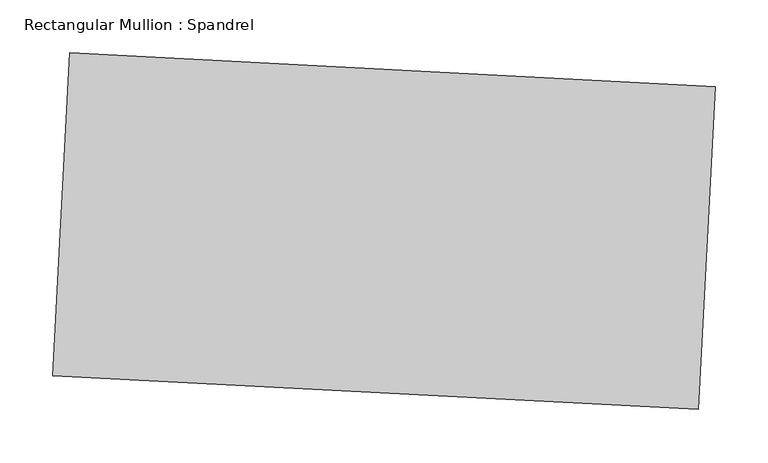
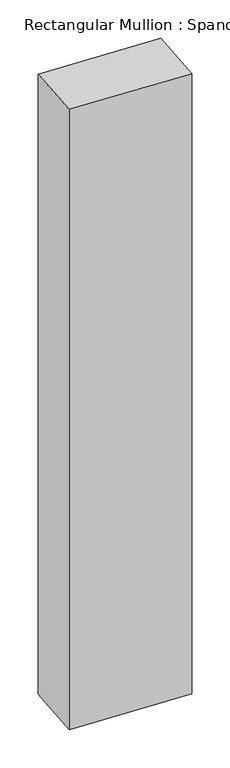
"""IFC4 building model written with IfcOpenShell, lengths in millimetres: member geometry, Rectangular Mullion : Spandrel."""

import ifcopenshell
import ifcopenshell.guid

model = None  # the IFC model being written
_history = None  # IfcOwnerHistory: only IFC2X3 demands one
_inside = {}  # id of a spatial element -> (the spatial element, [elements in it])
_under = {}  # id of a project, library or spatial element -> (it, [spatial elements below it])
_declared = {}  # id of a project -> (the project, [libraries it declares])
_typed = {}  # id of a type object -> (the type object, [elements of that type])
_made_of = {}  # id of a material, layer set ... -> (it, [elements and type objects made of it])


def new_model(schema):
    """Start an empty IFC model of exactly this schema.

    Asked for "IFC4X3", IfcOpenShell would pick the latest addendum, in which some entities
    have other attributes; the version numbers below select the first issue.
    IFC2X3 requires an IfcOwnerHistory on every rooted entity: one is made here for all.
    """
    global model, _history
    if schema == "IFC4X3":
        model = ifcopenshell.file(schema_version=(4, 3, 0, 0))
    else:
        model = ifcopenshell.file(schema=schema)
    _inside.clear()
    _under.clear()
    _declared.clear()
    _typed.clear()
    _made_of.clear()
    _history = None
    if model.schema == "IFC2X3":
        org = make("IfcOrganization", Name="unknown")
        user = make(
            "IfcPersonAndOrganization",
            ThePerson=make("IfcPerson", FamilyName="unknown"),
            TheOrganization=org,
        )
        app = make(
            "IfcApplication",
            ApplicationDeveloper=org,
            Version="unknown",
            ApplicationFullName="unknown",
            ApplicationIdentifier="unknown",
        )
        _history = make(
            "IfcOwnerHistory",
            OwningUser=user,
            OwningApplication=app,
            ChangeAction="ADDED",
            CreationDate=0,
        )
    return model


def make(cls, **values):
    """One entity of the class cls with the attributes given. An attribute that is None is left unset."""
    return model.create_entity(
        cls, **{name: value for name, value in values.items() if value is not None}
    )


def rooted(cls, **values):
    """An entity with a GlobalId (a new one), such as an element, a storey or a relation."""
    return make(cls, GlobalId=ifcopenshell.guid.new(), OwnerHistory=_history, **values)


def si_unit(unit_type, name, prefix=None):
    """IfcSIUnit, for example si_unit("LENGTHUNIT", "METRE", prefix="MILLI")."""
    return make("IfcSIUnit", UnitType=unit_type, Prefix=prefix, Name=name)


def assignment(units):
    """IfcUnitAssignment: the units of a project."""
    return None if units is None else make("IfcUnitAssignment", Units=units)


def point(xyz):
    """IfcCartesianPoint."""
    return None if xyz is None else make("IfcCartesianPoint", Coordinates=xyz)


def direction(xyz):
    """IfcDirection."""
    return None if xyz is None else make("IfcDirection", DirectionRatios=xyz)


def frame(location, z_axis=None, x_axis=None):
    """IfcAxis2Placement3D, a coordinate frame: its origin and axes. An axis left out is left unset."""
    return make(
        "IfcAxis2Placement3D",
        Location=point(location),
        Axis=direction(z_axis),
        RefDirection=direction(x_axis),
    )


def origin():
    """The frame at (0, 0, 0) with its axes left unset."""
    return frame((0.0, 0.0, 0.0))


def place(relative_to, where):
    """IfcLocalPlacement: puts the frame where relative to a parent placement (None: the world)."""
    return make(
        "IfcLocalPlacement", PlacementRelTo=relative_to, RelativePlacement=where
    )


def context(
    kind, dimensions, precision=None, world=None, true_north=None, identifier=None
):
    """IfcGeometricRepresentationContext, for example the 3D "Model" context."""
    return make(
        "IfcGeometricRepresentationContext",
        ContextIdentifier=identifier,
        ContextType=kind,
        CoordinateSpaceDimension=dimensions,
        Precision=precision,
        WorldCoordinateSystem=world,
        TrueNorth=true_north,
    )


def project(units=None, contexts=None):
    """IfcProject with its units and contexts."""
    return rooted(
        "IfcProject",
        Name="project",
        RepresentationContexts=contexts,
        UnitsInContext=assignment(units),
    )


def spatial(cls, under=None, at=None, **own):
    """A site, building, storey or space (cls), placed at a placement, below another one or the project."""
    s = rooted(cls, ObjectPlacement=at, **own)
    if under is not None:
        _under.setdefault(under.id(), (under, []))[1].append(s)
    return s


def polyline(points):
    """IfcPolyline through the points."""
    return make("IfcPolyline", Points=[point(p) for p in points])


def outline(outer, holes=None, kind="AREA"):
    """IfcArbitraryClosedProfileDef: a profile drawn as a closed curve; with holes, ...WithVoids."""
    if holes is None:
        return make("IfcArbitraryClosedProfileDef", ProfileType=kind, OuterCurve=outer)
    return make(
        "IfcArbitraryProfileDefWithVoids",
        ProfileType=kind,
        OuterCurve=outer,
        InnerCurves=holes,
    )


def extrude(swept, where, along, depth):
    """IfcExtrudedAreaSolid: the profile swept, set in the frame where, extruded along a direction by depth."""
    return make(
        "IfcExtrudedAreaSolid",
        SweptArea=swept,
        Position=where,
        ExtrudedDirection=direction(along),
        Depth=depth,
    )


def shape(context_of_items, identifier, shape_type, items):
    """IfcShapeRepresentation: the items that make up one representation, for example the "Body"."""
    return make(
        "IfcShapeRepresentation",
        ContextOfItems=context_of_items,
        RepresentationIdentifier=identifier,
        RepresentationType=shape_type,
        Items=items,
    )


def source(mapping_origin, context_of_items, identifier, shape_type, items):
    """IfcRepresentationMap: a shape defined once, which mapped items show again and again."""
    return make(
        "IfcRepresentationMap",
        MappingOrigin=mapping_origin,
        MappedRepresentation=shape(context_of_items, identifier, shape_type, items),
    )


def transform(
    local_origin,
    x_axis=None,
    y_axis=None,
    z_axis=None,
    scale=None,
    scale2=None,
    scale3=None,
    uniform=True,
):
    """IfcCartesianTransformationOperator3D, or its non-uniform kind. x_axis, y_axis, z_axis: its Axis1, 2, 3."""
    if uniform:
        return make(
            "IfcCartesianTransformationOperator3D",
            Axis1=direction(x_axis),
            Axis2=direction(y_axis),
            LocalOrigin=point(local_origin),
            Scale=scale,
            Axis3=direction(z_axis),
        )
    return make(
        "IfcCartesianTransformationOperator3DnonUniform",
        Axis1=direction(x_axis),
        Axis2=direction(y_axis),
        LocalOrigin=point(local_origin),
        Scale=scale,
        Axis3=direction(z_axis),
        Scale2=scale2,
        Scale3=scale3,
    )


def mapped(mapping_source, mapping_target):
    """IfcMappedItem: shows the shape of a source again, moved by a transform."""
    return make(
        "IfcMappedItem", MappingSource=mapping_source, MappingTarget=mapping_target
    )


def made_of(thing, what):
    """Note that an element or type object is made of a material, layer set ...; save() writes the relation."""
    if what is not None:
        _made_of.setdefault(what.id(), (what, []))[1].append(thing)
    return thing


def element(
    cls,
    number,
    at=None,
    inside=None,
    cuts=None,
    type_object=None,
    material=None,
    context=None,
    identifier="Body",
    shape_type=None,
    held_by="IfcProductDefinitionShape",
    body=None,
    shapes=None,
    **own,
):
    """One element of the class cls, such as IfcWall. Its Tag is "e" and its number.

    at: its placement. inside: the storey or other place that contains it. cuts: it is an
    opening in that element (IfcRelVoidsElement). A single representation is given by context,
    identifier, shape_type and body (its items); several are given by shapes. held_by: the class
    of the entity that holds the representations. save() writes the other relations.
    """
    e = rooted(cls, Tag="e%d" % number, ObjectPlacement=at, **own)
    if body is not None:
        shapes = [shape(context, identifier, shape_type, body)]
    if shapes is not None:
        e.Representation = make(held_by, Representations=shapes)
    if inside is not None:
        _inside.setdefault(inside.id(), (inside, []))[1].append(e)
    if cuts is not None:
        rooted(
            "IfcRelVoidsElement", RelatingBuildingElement=cuts, RelatedOpeningElement=e
        )
    if type_object is not None:
        _typed.setdefault(type_object.id(), (type_object, []))[1].append(e)
    return made_of(e, material)


def aggregate(whole, parts):
    """IfcRelAggregates: a whole, such as a stair, and the parts it consists of."""
    return rooted("IfcRelAggregates", RelatingObject=whole, RelatedObjects=parts)


def save(model, path):
    """Write the relations noted so far, then the file.

    IfcRelAggregates (storeys below a building ...), IfcRelContainedInSpatialStructure (elements
    in a storey), IfcRelDefinesByType, IfcRelAssociatesMaterial and IfcRelDeclares: one each for
    every whole, place, type object, material and project.
    """
    for whole, parts in _under.values():
        aggregate(whole, parts)
    for where, things in _inside.values():
        rooted(
            "IfcRelContainedInSpatialStructure",
            RelatedElements=things,
            RelatingStructure=where,
        )
    for kind, things in _typed.values():
        rooted("IfcRelDefinesByType", RelatedObjects=things, RelatingType=kind)
    for what, things in _made_of.values():
        rooted("IfcRelAssociatesMaterial", RelatedObjects=things, RelatingMaterial=what)
    for by, libraries in _declared.values():
        rooted("IfcRelDeclares", RelatingContext=by, RelatedDefinitions=libraries)
    model.write(path)


def rectangular_mullion_spandrel_e01d9ec2(model_context):
    return source(origin(), model_context, "Body", "SweptSolid", [
        extrude(outline(polyline([(312.3582819, 136.2391416), (296.4062825, -168.1431406), (-312.3582819, -136.2391416), (-296.4062825, 168.1431406), (312.3582819, 136.2391416)])), frame((0.0, 0.0, -3352.8), z_axis=(0.0, 0.0, 1.0), x_axis=(1.0, 0.0, 0.0)), (0.0, 0.0, 1.0), 3352.8),
    ])


if __name__ == "__main__":
    model = new_model("IFC4")
    model_context = context("Model", 3, world=origin())
    ifc_project = project(units=[si_unit("LENGTHUNIT", "METRE", prefix="MILLI")], contexts=[model_context])
    site = spatial("IfcSite", under=ifc_project)
    building = spatial("IfcBuilding", under=site)
    placement = place(None, origin())
    rectangular_mullion_spandrel_shape = rectangular_mullion_spandrel_e01d9ec2(model_context)
    element("IfcMember", 1, ObjectType="Rectangular Mullion : Spandrel", at=placement, inside=building, context=model_context, shape_type="MappedRepresentation", body=[
        mapped(rectangular_mullion_spandrel_shape, transform((0.0, 0.0, 0.0), x_axis=(1.0, 0.0, 0.0), y_axis=(0.0, 1.0, 0.0), z_axis=(0.0, 0.0, 1.0))),
    ])
    save(model, "model.ifc")

# Revit data of these elements
# Type "Rectangular Mullion : Spandrel"
#   built-in parameter 1007304 = 1 (stored number, unit not read)
#   built-in parameter 1007301 = 1 (stored number, unit not read)
#   built-in parameter 1007300 = 1 (stored number, unit not read)
# Element 1 (IfcMember, "Rectangular Mullion : Spandrel")
#   Materials on its faces: "Aluminum"
# Materials
#   "Aluminum": class "Metal", colour RGB 247 247 247, transparency 0, Description = "Aluminum 6061", Cost = 0
